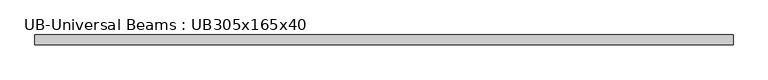
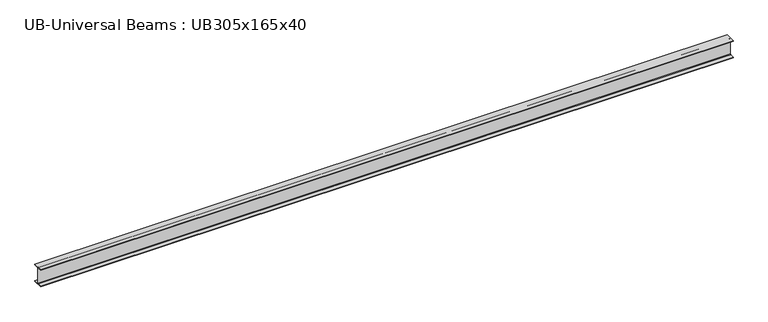
"""IFC4 building model written with IfcOpenShell, lengths in millimetres: member geometry, UB-Universal Beams : UB305x165x40."""

from ifc_helpers import new_model, si_unit, point, frame, frame_2d, origin, place, context, project, spatial, polyline, circle_curve, trimmed, segment, composite_curve, outline, extrude, source, transform, mapped, element, save


def ub_universal_beams_ub305x165x40_3335d084(model_context):
    return source(origin(), model_context, "Body", "SweptSolid", [
        extrude(outline(composite_curve([segment(polyline([(82.5, -141.5), (82.5, -151.7), (-82.5, -151.7), (-82.5, -141.5), (-11.9, -141.5)]), True, "CONTINUOUS"), segment(trimmed(circle_curve(frame_2d((-11.9, -132.6)), 8.9), [point((-11.9, -141.5))], [point((-3.0, -132.6))], True, "CARTESIAN"), True, "CONTINUOUS"), segment(polyline([(-3.0, -132.6), (-3.0, 132.6)]), True, "CONTINUOUS"), segment(trimmed(circle_curve(frame_2d((-11.9, 132.6)), 8.9), [point((-3.0, 132.6))], [point((-11.9, 141.5))], True, "CARTESIAN"), True, "CONTINUOUS"), segment(polyline([(-11.9, 141.5), (-82.5, 141.5), (-82.5, 151.7), (82.5, 151.7), (82.5, 141.5), (11.9, 141.5)]), True, "CONTINUOUS"), segment(trimmed(circle_curve(frame_2d((11.9, 132.6)), 8.9), [point((11.9, 141.5))], [point((3.0, 132.6))], True, "CARTESIAN"), True, "CONTINUOUS"), segment(polyline([(3.0, 132.6), (3.0, -132.6)]), True, "CONTINUOUS"), segment(trimmed(circle_curve(frame_2d((11.9, -132.6)), 8.9), [point((3.0, -132.6))], [point((11.9, -141.5))], True, "CARTESIAN"), True, "CONTINUOUS"), segment(polyline([(11.9, -141.5), (82.5, -141.5)]), True, "CONTINUOUS")], self_intersect=False)), frame((-5955.8, 0.0, 0.0), z_axis=(1.0, 0.0, 0.0), x_axis=(0.0, 1.0, 0.0)), (0.0, 0.0, 1.0), 11638.4),
    ])


if __name__ == "__main__":
    model = new_model("IFC4")
    model_context = context("Model", 3, world=origin())
    ifc_project = project(units=[si_unit("LENGTHUNIT", "METRE", prefix="MILLI")], contexts=[model_context])
    site = spatial("IfcSite", under=ifc_project)
    building = spatial("IfcBuilding", under=site)
    placement = place(None, origin())
    ub_universal_beams_ub305x165x40_shape = ub_universal_beams_ub305x165x40_3335d084(model_context)
    element("IfcMember", 1, ObjectType="UB-Universal Beams : UB305x165x40", at=placement, inside=building, context=model_context, shape_type="MappedRepresentation", body=[
        mapped(ub_universal_beams_ub305x165x40_shape, transform((0.0, 0.0, 0.0), x_axis=(1.0, 0.0, 0.0), y_axis=(0.0, 1.0, 0.0), z_axis=(0.0, 0.0, 1.0))),
    ])
    save(model, "model.ifc")

# Revit data of these elements
# Type "UB-Universal Beams : UB305x165x40"
#   Section Name Key = "UB305X165X40"
#   Width = 16.5 cm
#   Web Thickness = 0.6 cm
#   Web Fillet = 0.89 cm
#   Warping Constant = 164000.0 cm⁶
#   Torsional Moment of Inertia = 14.70 cm⁴
#   Section Area = 51.3 cm²
#   Plastic Modulus weak axis = 142.0 cm³
#   Plastic Modulus strong axis = 623.0 cm³
#   Nominal Weight = 40.2999 kgf/m
#   Moment of Inertia weak axis = 764.00 cm⁴
#   Moment of Inertia strong axis = 8503.00 cm⁴
#   Height = 30.34 cm
#   Flange Thickness = 1.02 cm
#   Elastic Modulus weak axis = 92.6 cm³
#   Elastic Modulus strong axis = 560.0 cm³
#   Centroid Vertical = 15.17 cm
#   Centroid Horizontal = 8.25 cm
#   Bolt Spacing = 9.0 cm
#   Length [instance default] = 1500 mm
#   Structural Material [instance default] = Metal - Steel 43-275
#   Type Comments = ""
#   Assembly Code = ""
# Element 1 (IfcMember, "UB-Universal Beams : UB305x165x40")
#   Materials on its faces: "Metal - Steel 43-275"
# Materials
#   "Metal - Steel 43-275": class "Metal", colour RGB 247 247 247, transparency 0, Cost = 0
